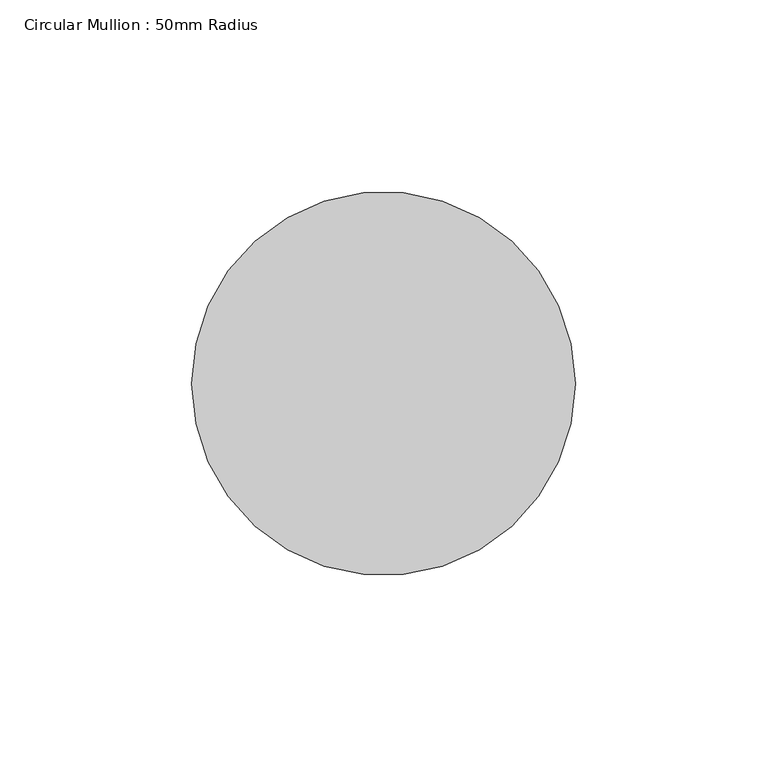
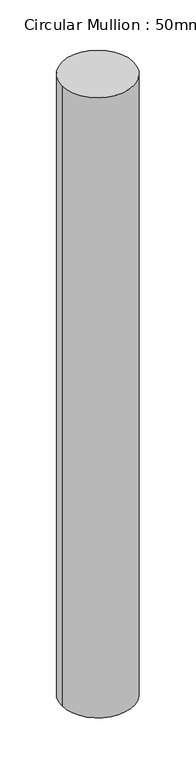
"""IFC4 building model written with IfcOpenShell, lengths in millimetres: member geometry, Circular Mullion : 50mm Radius."""

from ifc_helpers import new_model, si_unit, point, frame, origin, origin_2d, place, context, project, spatial, circle_curve, trimmed, segment, composite_curve, outline, extrude, source, transform, mapped, element, save


def circular_mullion_50mm_radius_08e6924e(model_context):
    return source(origin(), model_context, "Body", "SweptSolid", [
        extrude(outline(composite_curve([segment(trimmed(circle_curve(origin_2d(), 50.0), [point((50.0, 0.0))], [point((-50.0, 0.0))], False, "CARTESIAN"), True, "CONTINUOUS"), segment(trimmed(circle_curve(origin_2d(), 50.0), [point((-50.0, 0.0))], [point((50.0, 0.0))], False, "CARTESIAN"), True, "CONTINUOUS")], self_intersect=False)), frame((0.0, 0.0, -913.8158577), z_axis=(0.0, 0.0, 1.0), x_axis=(1.0, 0.0, 0.0)), (0.0, 0.0, 1.0), 913.8158577),
    ])


if __name__ == "__main__":
    model = new_model("IFC4")
    model_context = context("Model", 3, world=origin())
    ifc_project = project(units=[si_unit("LENGTHUNIT", "METRE", prefix="MILLI")], contexts=[model_context])
    site = spatial("IfcSite", under=ifc_project)
    building = spatial("IfcBuilding", under=site)
    placement = place(None, origin())
    circular_mullion_50mm_radius_shape = circular_mullion_50mm_radius_08e6924e(model_context)
    element("IfcMember", 1, ObjectType="Circular Mullion : 50mm Radius", at=placement, inside=building, context=model_context, shape_type="MappedRepresentation", body=[
        mapped(circular_mullion_50mm_radius_shape, transform((0.0, 0.0, 0.0), x_axis=(1.0, 0.0, 0.0), y_axis=(0.0, 1.0, 0.0), z_axis=(0.0, 0.0, 1.0))),
    ])
    save(model, "model.ifc")

# Revit data of these elements
# Type "Circular Mullion : 50mm Radius"
#   built-in parameter 1007350 = 0.164042 (stored number, unit not read)
# Element 1 (IfcMember, "Circular Mullion : 50mm Radius")
#   Materials on its faces: "Aluminium"
# Materials
#   "Aluminium": class "Metal", colour RGB 247 247 247, transparency 0, Description = "Aluminium 6061", Cost = 0
